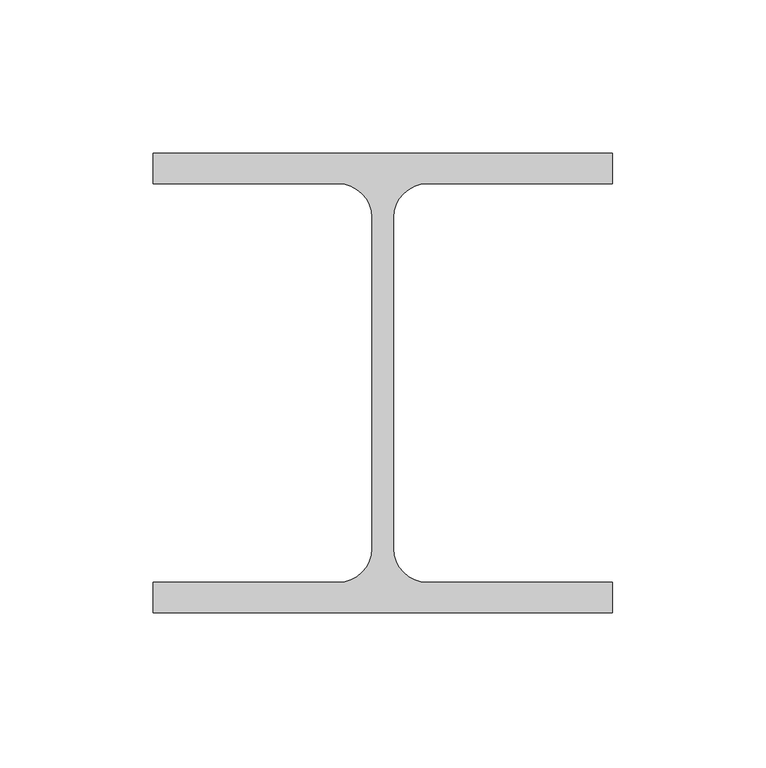
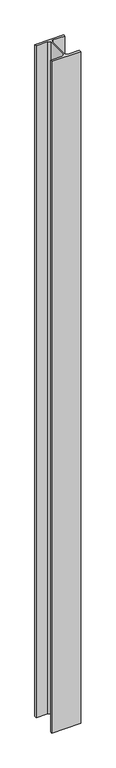
"""IFC4 building model written with IfcOpenShell, lengths in millimetres: column geometry, 0912_Steel Column_H_KSD3502 : H_SC_ASC_H-150x150x7x10."""

from ifc_helpers import new_model, si_unit, point, frame, frame_2d, origin, place, context, project, spatial, polyline, circle_curve, trimmed, segment, composite_curve, outline, extrude, source, transform, mapped, element, save


def column_3e22cd7b(model_context):
    return source(origin(), model_context, "Body", "SweptSolid", [
        extrude(outline(composite_curve([segment(polyline([(75.0, 75.0), (75.0, 65.0), (14.5, 65.0)]), True, "CONTINUOUS"), segment(trimmed(circle_curve(frame_2d((14.5, 54.0)), 11.0), [point((14.5, 65.0))], [point((3.5, 54.0))], True, "CARTESIAN"), True, "CONTINUOUS"), segment(polyline([(3.5, 54.0), (3.5, -54.0)]), True, "CONTINUOUS"), segment(trimmed(circle_curve(frame_2d((14.5, -54.0)), 11.0), [point((3.5, -54.0))], [point((14.5, -65.0))], True, "CARTESIAN"), True, "CONTINUOUS"), segment(polyline([(14.5, -65.0), (75.0, -65.0), (75.0, -75.0), (-75.0, -75.0), (-75.0, -65.0), (-14.5, -65.0)]), True, "CONTINUOUS"), segment(trimmed(circle_curve(frame_2d((-14.5, -54.0)), 11.0), [point((-14.5, -65.0))], [point((-3.5, -54.0))], True, "CARTESIAN"), True, "CONTINUOUS"), segment(polyline([(-3.5, -54.0), (-3.5, 54.0)]), True, "CONTINUOUS"), segment(trimmed(circle_curve(frame_2d((-14.5, 54.0)), 11.0), [point((-3.5, 54.0))], [point((-14.5, 65.0))], True, "CARTESIAN"), True, "CONTINUOUS"), segment(polyline([(-14.5, 65.0), (-75.0, 65.0), (-75.0, 75.0), (75.0, 75.0)]), True, "CONTINUOUS")], self_intersect=False)), frame((0.0, 0.0, 599.9720055), z_axis=(0.0, 0.0, 1.0), x_axis=(1.0, 0.0, 0.0)), (0.0, 0.0, 1.0), 3678.0),
    ])


if __name__ == "__main__":
    model = new_model("IFC4")
    model_context = context("Model", 3, world=origin())
    ifc_project = project(units=[si_unit("LENGTHUNIT", "METRE", prefix="MILLI")], contexts=[model_context])
    site = spatial("IfcSite", under=ifc_project)
    building = spatial("IfcBuilding", under=site)
    placement = place(None, origin())
    column_shape = column_3e22cd7b(model_context)
    element("IfcColumn", 1, ObjectType="0912_Steel Column_H_KSD3502 : H_SC_ASC_H-150x150x7x10", at=placement, inside=building, context=model_context, shape_type="MappedRepresentation", body=[
        mapped(column_shape, transform((0.0, 0.0, 0.0), x_axis=(1.0, 0.0, 0.0), y_axis=(0.0, 1.0, 0.0), z_axis=(0.0, 0.0, 1.0))),
    ])
    save(model, "model.ifc")

# Revit data of these elements
# Type "0912_Steel Column_H_KSD3502 : H_SC_ASC_H-150x150x7x10"
#   H_WM Code_1 = "S01AA002-00001 | Main Steel Structure Fabrication Work | Shelter/Building | Medium Steel - Standard (90KG/M>Weight≥30KG/M) | Material: (   )"
#   H_WM Code_2 = "S03AA028-00001 | Main Steel Structure Erection Work | Shelter/Building | Medium Steel (90KG/M>Weight≥30KG/M) | Material: (   )"
#   H_WM Code_3 = "S01AA010-00001 | Main Steel Structure Fabrication Work | Shelter/Building | Steel Painting/Coating | for Non-Fireproofed Steel Surface, Surface Preparation, Primer, Second & Final Coat | Material: (   )"
#   H_Q'ty Cal Type Tag = "SC-Q2"
#   Width = 15.0 cm
#   Web Thickness = 0.7 cm
#   Web Fillet = 1.1 cm
#   Warping Constant = 27562.5 cm⁶
#   Torsional Moment of Inertia = 11.6007 cm⁴
#   Section Area = 40.14 cm²
#   Plastic Modulus weak axis = 115.0 cm³
#   Plastic Modulus strong axis = 246.0 cm³
#   Perimeter = 0.87 m²/m
#   Nominal Weight = 31.50 kgf/m
#   Moment of Inertia weak axis = 563.00 cm⁴
#   Moment of Inertia strong axis = 1640.00 cm⁴
#   Height = 15.0 cm
#   Flange Thickness = 1.0 cm
#   Elastic Modulus weak axis = 75.1 cm³
#   Elastic Modulus strong axis = 219.0 cm³
#   Centroid Vertical = 7.5 cm
#   Centroid Horizontal = 7.5 cm
#   Structural Material [instance default] = Steel, 45-345
#   Section Name Key = ""
#   Bolt Spacing = 0
#   Assembly Code = ""
# Element 1 (IfcColumn, "0912_Steel Column_H_KSD3502 : H_SC_ASC_H-150x150x7x10")
#   Structural Material = A03AD029-00005_Anchor Bolt (Installation only)_M24
#   Materials on its faces: "A03AD029-00005_Anchor Bolt (Installation only)_M24"
# Materials
#   "Steel, 45-345": class "Metal", colour RGB 189 187 185, transparency 0, Description = "Steel 345 MPa", Cost = 0
#   "A03AD029-00005_Anchor Bolt (Installation only)_M24": class "Unassigned", colour RGB 84 83 81, transparency 0, Cost = 0
